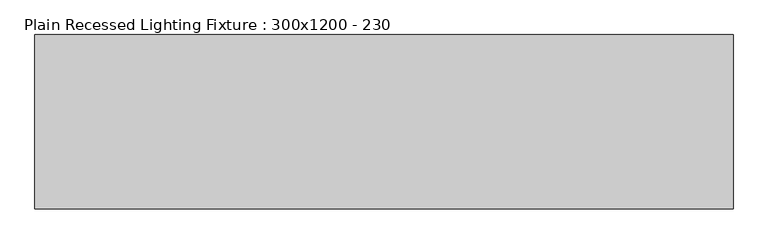
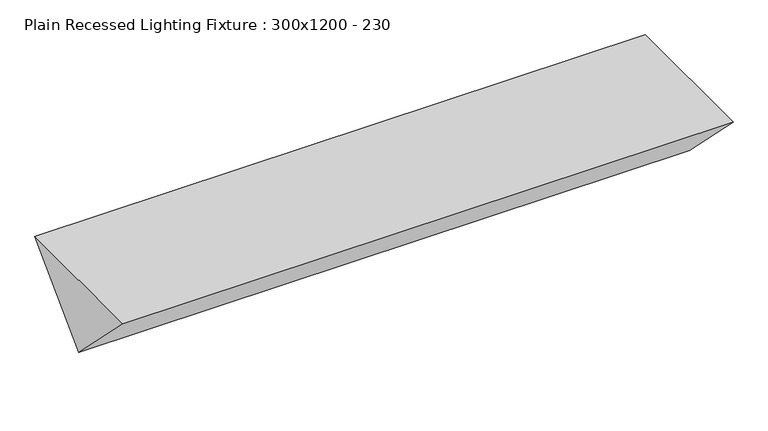
"""IFC4 building model written with IfcOpenShell, lengths in millimetres: light fixture geometry, Plain Recessed Lighting Fixture : 300x1200 - 230."""

from ifc_helpers import new_model, si_unit, frame, origin, place, context, project, spatial, polyline, outline, extrude, source, transform, mapped, element, save


def plain_recessed_lighting_fixture_300x1200_230_e46e8774(model_context):
    return source(origin(), model_context, "Body", "SweptSolid", [
        extrude(outline(polyline([(-300.0, 0.0), (0.0, 0.0), (-150.0, -150.0), (-300.0, 0.0)])), frame((0.0, 0.0, 0.0), z_axis=(1.0, 0.0, 0.0), x_axis=(0.0, 1.0, 0.0)), (0.0, 0.0, 1.0), 1200.0),
    ])


if __name__ == "__main__":
    model = new_model("IFC4")
    model_context = context("Model", 3, world=origin())
    ifc_project = project(units=[si_unit("LENGTHUNIT", "METRE", prefix="MILLI")], contexts=[model_context])
    site = spatial("IfcSite", under=ifc_project)
    building = spatial("IfcBuilding", under=site)
    placement = place(None, origin())
    plain_recessed_lighting_fixture_300x1200_230_shape = plain_recessed_lighting_fixture_300x1200_230_e46e8774(model_context)
    element("IfcLightFixture", 1, ObjectType="Plain Recessed Lighting Fixture : 300x1200 - 230", at=placement, inside=building, context=model_context, shape_type="MappedRepresentation", body=[
        mapped(plain_recessed_lighting_fixture_300x1200_230_shape, transform((0.0, 0.0, 0.0), x_axis=(1.0, 0.0, 0.0), y_axis=(0.0, 1.0, 0.0), z_axis=(0.0, 0.0, 1.0))),
    ])
    save(model, "model.ifc")

# Revit data of these elements
# Type "Plain Recessed Lighting Fixture : 300x1200 - 230"
#   Photometric Web File = "1x42A12.ies"
#   Width = 300 mm
#   Wattage = 64 W
#   built-in parameter 1150110 = 1 (stored number, unit not read)
#   built-in parameter 1150109 = 1 (stored number, unit not read)
#   built-in parameter 1150113 = 1 (stored number, unit not read)
#   Tilt Angle = -90.00°
#   Lumens = 5699.84 lm
#   built-in parameter 1114217 = 0.88 (stored number, unit not read)
#   built-in parameter 1150115 = 1 (stored number, unit not read)
#   built-in parameter 1150105 = 453.579 (stored number, unit not read)
#   Length = 1200 mm
#   built-in parameter 1150112 = 1 (stored number, unit not read)
#   built-in parameter 1150114 = 1 (stored number, unit not read)
#   built-in parameter 1150107 = 4230 (stored number, unit not read)
#   built-in parameter 1150106 = 4.53579 (stored number, unit not read)
#   Emit from Rectangle Width = 300 mm
#   Emit from Rectangle Length = 1200 mm
#   built-in parameter 1150104 = 8.27394 (stored number, unit not read)
#   Depth = 150 mm
#   Default Elevation = 2000 mm
#   Ballast Voltage = 230 V
#   built-in parameter 1114218 = 0.88 (stored number, unit not read)
#   built-in parameter 1150133 = 10 (stored number, unit not read)
#   Apparent Load = 64 VA
#   built-in parameter 1150134 = 8
#   built-in parameter 1150137 = 1
#   Color Filter = 16777215
#   built-in parameter 1140040 [instance default] = 1
#   Load Classification = Lighting - Dwelling Unit
#   Emit Shape Visible in Rendering = no
#   Dimming Lamp Color Temperature Shift = (empty or 0)
#   Assembly Code = ""
